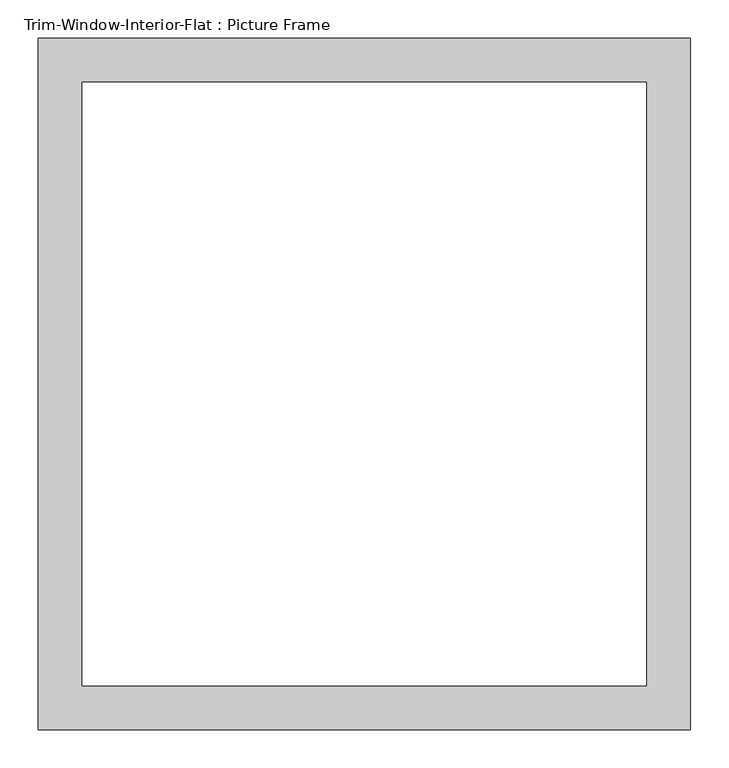
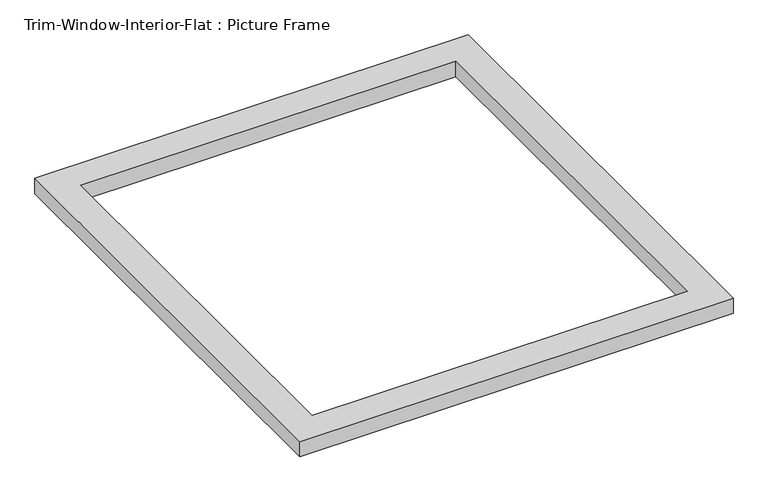
"""IFC4 building model written with IfcOpenShell, lengths in millimetres: proxy geometry, Trim-Window-Interior-Flat : Picture Frame."""

from ifc_helpers import new_model, si_unit, origin, origin_with_axes, place, context, project, spatial, polyline, outline, extrude, source, transform, mapped, element, save


def trim_window_interior_flat_picture_frame_4614366b(model_context):
    return source(origin(), model_context, "Body", "SweptSolid", [
        extrude(outline(polyline([(425.45, 44.45), (425.45, -857.25), (-425.45, -857.25), (-425.45, 44.45), (425.45, 44.45)]), holes=[polyline([(368.3, -12.7), (-368.3, -12.7), (-368.3, -800.1), (368.3, -800.1), (368.3, -12.7)])]), origin_with_axes(), (0.0, 0.0, 1.0), 31.75),
    ])


if __name__ == "__main__":
    model = new_model("IFC4")
    model_context = context("Model", 3, world=origin())
    ifc_project = project(units=[si_unit("LENGTHUNIT", "METRE", prefix="MILLI")], contexts=[model_context])
    site = spatial("IfcSite", under=ifc_project)
    building = spatial("IfcBuilding", under=site)
    placement = place(None, origin())
    trim_window_interior_flat_picture_frame_shape = trim_window_interior_flat_picture_frame_4614366b(model_context)
    element("IfcBuildingElementProxy", 1, Name="Trim-Window-Interior-Flat : Picture Frame", ObjectType="Trim-Window-Interior-Flat : Picture Frame", at=placement, inside=building, context=model_context, shape_type="MappedRepresentation", body=[
        mapped(trim_window_interior_flat_picture_frame_shape, transform((0.0, 0.0, 0.0), x_axis=(1.0, 0.0, 0.0), y_axis=(0.0, 1.0, 0.0), z_axis=(0.0, 0.0, 1.0))),
    ])
    save(model, "model.ifc")

# Revit data of these elements
# Type "Trim-Window-Interior-Flat : Picture Frame"
#   Trim Thickness_Picture Frame = 0' - 1 1/4"
#   Trim Width = 0' - 2 1/4"
#   Trim Thickness_with Sill = 0' - 0 3/4"
#   Sill Thickness = 0' - 1 1/4"
#   Opening Width [instance default] = 2' - 0"
#   Opening Height [instance default] = 3' - 0"
#   Default Elevation = 4' - 0"
#   Sill = no
#   Picture Frame = yes
#   Trim Material [instance default] = none
# Element 1 (IfcBuildingElementProxy, "Trim-Window-Interior-Flat : Picture Frame")
#   Opening Width = 2' - 6"
#   Opening Height = 2' - 8"
#   Trim Material = Wood - Stained
#   Materials on its faces: "Wood - Stained"
# Materials
#   "Wood - Stained": class "Wood", colour RGB 224 178 126, transparency 0, Cost = 0
